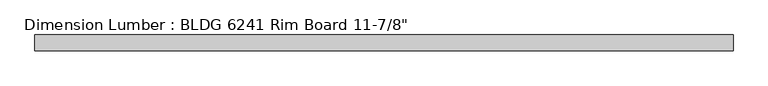
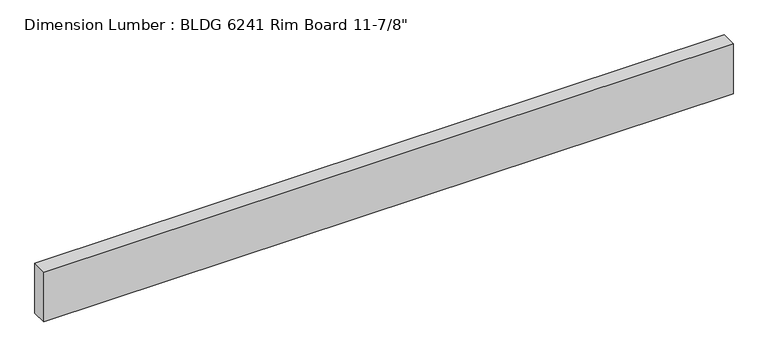
"""IFC4 building model written with IfcOpenShell, lengths in millimetres: beam geometry."""

import ifcopenshell
import ifcopenshell.guid

model = None  # the IFC model being written
_history = None  # IfcOwnerHistory: only IFC2X3 demands one
_inside = {}  # id of a spatial element -> (the spatial element, [elements in it])
_under = {}  # id of a project, library or spatial element -> (it, [spatial elements below it])
_declared = {}  # id of a project -> (the project, [libraries it declares])
_typed = {}  # id of a type object -> (the type object, [elements of that type])
_made_of = {}  # id of a material, layer set ... -> (it, [elements and type objects made of it])


def new_model(schema):
    """Start an empty IFC model of exactly this schema.

    Asked for "IFC4X3", IfcOpenShell would pick the latest addendum, in which some entities
    have other attributes; the version numbers below select the first issue.
    IFC2X3 requires an IfcOwnerHistory on every rooted entity: one is made here for all.
    """
    global model, _history
    if schema == "IFC4X3":
        model = ifcopenshell.file(schema_version=(4, 3, 0, 0))
    else:
        model = ifcopenshell.file(schema=schema)
    _inside.clear()
    _under.clear()
    _declared.clear()
    _typed.clear()
    _made_of.clear()
    _history = None
    if model.schema == "IFC2X3":
        org = make("IfcOrganization", Name="unknown")
        user = make(
            "IfcPersonAndOrganization",
            ThePerson=make("IfcPerson", FamilyName="unknown"),
            TheOrganization=org,
        )
        app = make(
            "IfcApplication",
            ApplicationDeveloper=org,
            Version="unknown",
            ApplicationFullName="unknown",
            ApplicationIdentifier="unknown",
        )
        _history = make(
            "IfcOwnerHistory",
            OwningUser=user,
            OwningApplication=app,
            ChangeAction="ADDED",
            CreationDate=0,
        )
    return model


def make(cls, **values):
    """One entity of the class cls with the attributes given. An attribute that is None is left unset."""
    return model.create_entity(
        cls, **{name: value for name, value in values.items() if value is not None}
    )


def rooted(cls, **values):
    """An entity with a GlobalId (a new one), such as an element, a storey or a relation."""
    return make(cls, GlobalId=ifcopenshell.guid.new(), OwnerHistory=_history, **values)


def si_unit(unit_type, name, prefix=None):
    """IfcSIUnit, for example si_unit("LENGTHUNIT", "METRE", prefix="MILLI")."""
    return make("IfcSIUnit", UnitType=unit_type, Prefix=prefix, Name=name)


def assignment(units):
    """IfcUnitAssignment: the units of a project."""
    return None if units is None else make("IfcUnitAssignment", Units=units)


def point(xyz):
    """IfcCartesianPoint."""
    return None if xyz is None else make("IfcCartesianPoint", Coordinates=xyz)


def direction(xyz):
    """IfcDirection."""
    return None if xyz is None else make("IfcDirection", DirectionRatios=xyz)


def frame(location, z_axis=None, x_axis=None):
    """IfcAxis2Placement3D, a coordinate frame: its origin and axes. An axis left out is left unset."""
    return make(
        "IfcAxis2Placement3D",
        Location=point(location),
        Axis=direction(z_axis),
        RefDirection=direction(x_axis),
    )


def origin():
    """The frame at (0, 0, 0) with its axes left unset."""
    return frame((0.0, 0.0, 0.0))


def place(relative_to, where):
    """IfcLocalPlacement: puts the frame where relative to a parent placement (None: the world)."""
    return make(
        "IfcLocalPlacement", PlacementRelTo=relative_to, RelativePlacement=where
    )


def context(
    kind, dimensions, precision=None, world=None, true_north=None, identifier=None
):
    """IfcGeometricRepresentationContext, for example the 3D "Model" context."""
    return make(
        "IfcGeometricRepresentationContext",
        ContextIdentifier=identifier,
        ContextType=kind,
        CoordinateSpaceDimension=dimensions,
        Precision=precision,
        WorldCoordinateSystem=world,
        TrueNorth=true_north,
    )


def project(units=None, contexts=None):
    """IfcProject with its units and contexts."""
    return rooted(
        "IfcProject",
        Name="project",
        RepresentationContexts=contexts,
        UnitsInContext=assignment(units),
    )


def spatial(cls, under=None, at=None, **own):
    """A site, building, storey or space (cls), placed at a placement, below another one or the project."""
    s = rooted(cls, ObjectPlacement=at, **own)
    if under is not None:
        _under.setdefault(under.id(), (under, []))[1].append(s)
    return s


def polyline(points):
    """IfcPolyline through the points."""
    return make("IfcPolyline", Points=[point(p) for p in points])


def outline(outer, holes=None, kind="AREA"):
    """IfcArbitraryClosedProfileDef: a profile drawn as a closed curve; with holes, ...WithVoids."""
    if holes is None:
        return make("IfcArbitraryClosedProfileDef", ProfileType=kind, OuterCurve=outer)
    return make(
        "IfcArbitraryProfileDefWithVoids",
        ProfileType=kind,
        OuterCurve=outer,
        InnerCurves=holes,
    )


def extrude(swept, where, along, depth):
    """IfcExtrudedAreaSolid: the profile swept, set in the frame where, extruded along a direction by depth."""
    return make(
        "IfcExtrudedAreaSolid",
        SweptArea=swept,
        Position=where,
        ExtrudedDirection=direction(along),
        Depth=depth,
    )


def shape(context_of_items, identifier, shape_type, items):
    """IfcShapeRepresentation: the items that make up one representation, for example the "Body"."""
    return make(
        "IfcShapeRepresentation",
        ContextOfItems=context_of_items,
        RepresentationIdentifier=identifier,
        RepresentationType=shape_type,
        Items=items,
    )


def source(mapping_origin, context_of_items, identifier, shape_type, items):
    """IfcRepresentationMap: a shape defined once, which mapped items show again and again."""
    return make(
        "IfcRepresentationMap",
        MappingOrigin=mapping_origin,
        MappedRepresentation=shape(context_of_items, identifier, shape_type, items),
    )


def transform(
    local_origin,
    x_axis=None,
    y_axis=None,
    z_axis=None,
    scale=None,
    scale2=None,
    scale3=None,
    uniform=True,
):
    """IfcCartesianTransformationOperator3D, or its non-uniform kind. x_axis, y_axis, z_axis: its Axis1, 2, 3."""
    if uniform:
        return make(
            "IfcCartesianTransformationOperator3D",
            Axis1=direction(x_axis),
            Axis2=direction(y_axis),
            LocalOrigin=point(local_origin),
            Scale=scale,
            Axis3=direction(z_axis),
        )
    return make(
        "IfcCartesianTransformationOperator3DnonUniform",
        Axis1=direction(x_axis),
        Axis2=direction(y_axis),
        LocalOrigin=point(local_origin),
        Scale=scale,
        Axis3=direction(z_axis),
        Scale2=scale2,
        Scale3=scale3,
    )


def mapped(mapping_source, mapping_target):
    """IfcMappedItem: shows the shape of a source again, moved by a transform."""
    return make(
        "IfcMappedItem", MappingSource=mapping_source, MappingTarget=mapping_target
    )


def made_of(thing, what):
    """Note that an element or type object is made of a material, layer set ...; save() writes the relation."""
    if what is not None:
        _made_of.setdefault(what.id(), (what, []))[1].append(thing)
    return thing


def element(
    cls,
    number,
    at=None,
    inside=None,
    cuts=None,
    type_object=None,
    material=None,
    context=None,
    identifier="Body",
    shape_type=None,
    held_by="IfcProductDefinitionShape",
    body=None,
    shapes=None,
    **own,
):
    """One element of the class cls, such as IfcWall. Its Tag is "e" and its number.

    at: its placement. inside: the storey or other place that contains it. cuts: it is an
    opening in that element (IfcRelVoidsElement). A single representation is given by context,
    identifier, shape_type and body (its items); several are given by shapes. held_by: the class
    of the entity that holds the representations. save() writes the other relations.
    """
    e = rooted(cls, Tag="e%d" % number, ObjectPlacement=at, **own)
    if body is not None:
        shapes = [shape(context, identifier, shape_type, body)]
    if shapes is not None:
        e.Representation = make(held_by, Representations=shapes)
    if inside is not None:
        _inside.setdefault(inside.id(), (inside, []))[1].append(e)
    if cuts is not None:
        rooted(
            "IfcRelVoidsElement", RelatingBuildingElement=cuts, RelatedOpeningElement=e
        )
    if type_object is not None:
        _typed.setdefault(type_object.id(), (type_object, []))[1].append(e)
    return made_of(e, material)


def aggregate(whole, parts):
    """IfcRelAggregates: a whole, such as a stair, and the parts it consists of."""
    return rooted("IfcRelAggregates", RelatingObject=whole, RelatedObjects=parts)


def save(model, path):
    """Write the relations noted so far, then the file.

    IfcRelAggregates (storeys below a building ...), IfcRelContainedInSpatialStructure (elements
    in a storey), IfcRelDefinesByType, IfcRelAssociatesMaterial and IfcRelDeclares: one each for
    every whole, place, type object, material and project.
    """
    for whole, parts in _under.values():
        aggregate(whole, parts)
    for where, things in _inside.values():
        rooted(
            "IfcRelContainedInSpatialStructure",
            RelatedElements=things,
            RelatingStructure=where,
        )
    for kind, things in _typed.values():
        rooted("IfcRelDefinesByType", RelatedObjects=things, RelatingType=kind)
    for what, things in _made_of.values():
        rooted("IfcRelAssociatesMaterial", RelatedObjects=things, RelatingMaterial=what)
    for by, libraries in _declared.values():
        rooted("IfcRelDeclares", RelatingContext=by, RelatedDefinitions=libraries)
    model.write(path)


def beam_dcf2d3fa(model_context):
    return source(origin(), model_context, "Body", "SweptSolid", [
        extrude(outline(polyline([(1927.225, 44.45), (1927.225, -44.45), (-2016.125, -44.45), (-2016.125, 44.45), (1927.225, 44.45)])), frame((0.0, 0.0, -150.8125), z_axis=(0.0, 0.0, 1.0), x_axis=(1.0, 0.0, 0.0)), (0.0, 0.0, 1.0), 301.625),
    ])


if __name__ == "__main__":
    model = new_model("IFC4")
    model_context = context("Model", 3, world=origin())
    ifc_project = project(units=[si_unit("LENGTHUNIT", "METRE", prefix="MILLI")], contexts=[model_context])
    site = spatial("IfcSite", under=ifc_project)
    building = spatial("IfcBuilding", under=site)
    placement = place(None, origin())
    beam_shape = beam_dcf2d3fa(model_context)
    element("IfcBeam", 1, ObjectType="Dimension Lumber : BLDG 6241 Rim Board 11-7/8\"", at=placement, inside=building, context=model_context, shape_type="MappedRepresentation", body=[
        mapped(beam_shape, transform((0.0, 0.0, 0.0), x_axis=(1.0, 0.0, 0.0), y_axis=(0.0, 1.0, 0.0), z_axis=(0.0, 0.0, 1.0))),
    ])
    save(model, "model.ifc")

# Revit data of these elements
# Type "Dimension Lumber : BLDG 6241 Rim Board 11-7/8\""
#   Assembly Code = "B10"
#   A = 0.273472 SF
#   Length [instance default] = 5' - 0"
#   b = 0' - 3 1/2"
#   d = 0' - 11 7/8"
#   Structural Material [instance default] = Softwood, Lumber
# Element 1 (IfcBeam, "Dimension Lumber : BLDG 6241 Rim Board 11-7/8\"")
#   Materials on its faces: "Softwood, Lumber"
# Materials
#   "Softwood, Lumber": class "Wood", colour RGB 223 192 134, transparency 0, Description = "Pinus Echinata", Cost = 0
